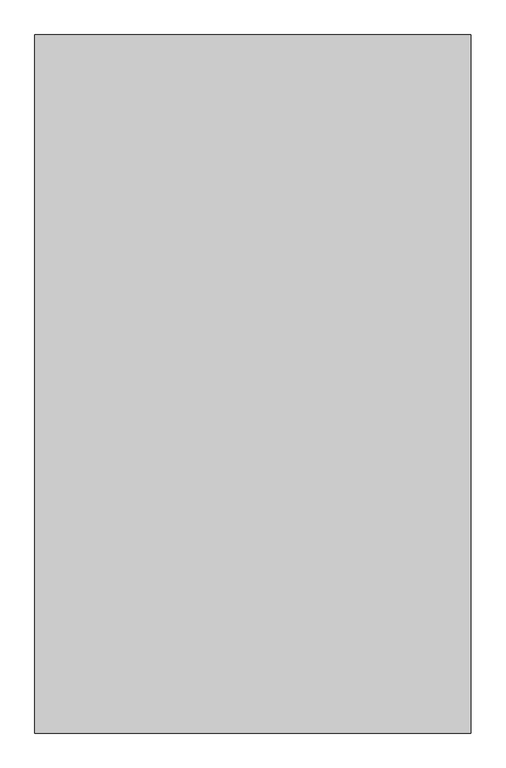
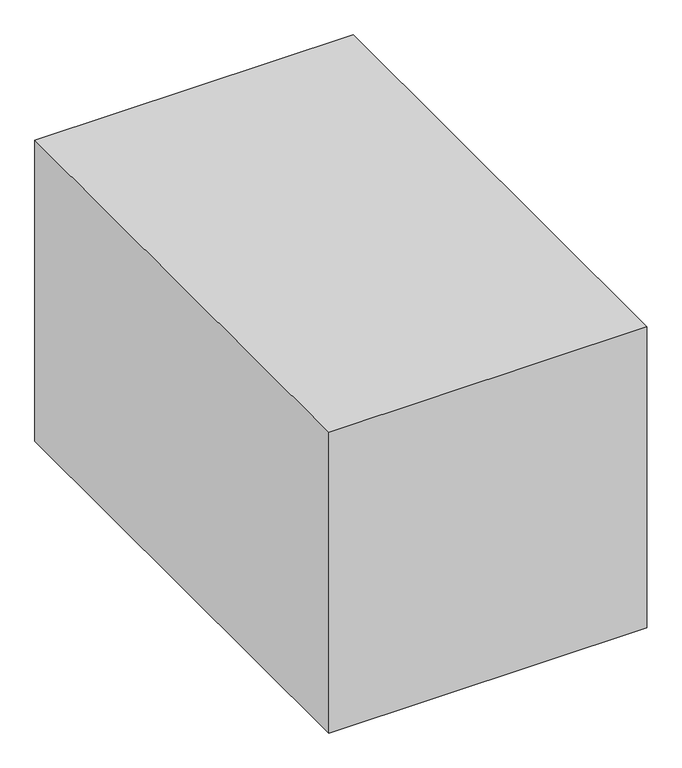
"""IFC4 building model written with IfcOpenShell, lengths in millimetres: proxy geometry, Space Planning Box_hec : Space Planning Box_hec."""

import ifcopenshell
import ifcopenshell.guid

model = None  # the IFC model being written
_history = None  # IfcOwnerHistory: only IFC2X3 demands one
_inside = {}  # id of a spatial element -> (the spatial element, [elements in it])
_under = {}  # id of a project, library or spatial element -> (it, [spatial elements below it])
_declared = {}  # id of a project -> (the project, [libraries it declares])
_typed = {}  # id of a type object -> (the type object, [elements of that type])
_made_of = {}  # id of a material, layer set ... -> (it, [elements and type objects made of it])


def new_model(schema):
    """Start an empty IFC model of exactly this schema.

    Asked for "IFC4X3", IfcOpenShell would pick the latest addendum, in which some entities
    have other attributes; the version numbers below select the first issue.
    IFC2X3 requires an IfcOwnerHistory on every rooted entity: one is made here for all.
    """
    global model, _history
    if schema == "IFC4X3":
        model = ifcopenshell.file(schema_version=(4, 3, 0, 0))
    else:
        model = ifcopenshell.file(schema=schema)
    _inside.clear()
    _under.clear()
    _declared.clear()
    _typed.clear()
    _made_of.clear()
    _history = None
    if model.schema == "IFC2X3":
        org = make("IfcOrganization", Name="unknown")
        user = make(
            "IfcPersonAndOrganization",
            ThePerson=make("IfcPerson", FamilyName="unknown"),
            TheOrganization=org,
        )
        app = make(
            "IfcApplication",
            ApplicationDeveloper=org,
            Version="unknown",
            ApplicationFullName="unknown",
            ApplicationIdentifier="unknown",
        )
        _history = make(
            "IfcOwnerHistory",
            OwningUser=user,
            OwningApplication=app,
            ChangeAction="ADDED",
            CreationDate=0,
        )
    return model


def make(cls, **values):
    """One entity of the class cls with the attributes given. An attribute that is None is left unset."""
    return model.create_entity(
        cls, **{name: value for name, value in values.items() if value is not None}
    )


def rooted(cls, **values):
    """An entity with a GlobalId (a new one), such as an element, a storey or a relation."""
    return make(cls, GlobalId=ifcopenshell.guid.new(), OwnerHistory=_history, **values)


def si_unit(unit_type, name, prefix=None):
    """IfcSIUnit, for example si_unit("LENGTHUNIT", "METRE", prefix="MILLI")."""
    return make("IfcSIUnit", UnitType=unit_type, Prefix=prefix, Name=name)


def assignment(units):
    """IfcUnitAssignment: the units of a project."""
    return None if units is None else make("IfcUnitAssignment", Units=units)


def point(xyz):
    """IfcCartesianPoint."""
    return None if xyz is None else make("IfcCartesianPoint", Coordinates=xyz)


def direction(xyz):
    """IfcDirection."""
    return None if xyz is None else make("IfcDirection", DirectionRatios=xyz)


def frame(location, z_axis=None, x_axis=None):
    """IfcAxis2Placement3D, a coordinate frame: its origin and axes. An axis left out is left unset."""
    return make(
        "IfcAxis2Placement3D",
        Location=point(location),
        Axis=direction(z_axis),
        RefDirection=direction(x_axis),
    )


def origin():
    """The frame at (0, 0, 0) with its axes left unset."""
    return frame((0.0, 0.0, 0.0))


def origin_with_axes():
    """The frame at (0, 0, 0) with the z axis (0, 0, 1) and the x axis (1, 0, 0) written out."""
    return frame((0.0, 0.0, 0.0), z_axis=(0.0, 0.0, 1.0), x_axis=(1.0, 0.0, 0.0))


def place(relative_to, where):
    """IfcLocalPlacement: puts the frame where relative to a parent placement (None: the world)."""
    return make(
        "IfcLocalPlacement", PlacementRelTo=relative_to, RelativePlacement=where
    )


def context(
    kind, dimensions, precision=None, world=None, true_north=None, identifier=None
):
    """IfcGeometricRepresentationContext, for example the 3D "Model" context."""
    return make(
        "IfcGeometricRepresentationContext",
        ContextIdentifier=identifier,
        ContextType=kind,
        CoordinateSpaceDimension=dimensions,
        Precision=precision,
        WorldCoordinateSystem=world,
        TrueNorth=true_north,
    )


def project(units=None, contexts=None):
    """IfcProject with its units and contexts."""
    return rooted(
        "IfcProject",
        Name="project",
        RepresentationContexts=contexts,
        UnitsInContext=assignment(units),
    )


def spatial(cls, under=None, at=None, **own):
    """A site, building, storey or space (cls), placed at a placement, below another one or the project."""
    s = rooted(cls, ObjectPlacement=at, **own)
    if under is not None:
        _under.setdefault(under.id(), (under, []))[1].append(s)
    return s


def polyline(points):
    """IfcPolyline through the points."""
    return make("IfcPolyline", Points=[point(p) for p in points])


def outline(outer, holes=None, kind="AREA"):
    """IfcArbitraryClosedProfileDef: a profile drawn as a closed curve; with holes, ...WithVoids."""
    if holes is None:
        return make("IfcArbitraryClosedProfileDef", ProfileType=kind, OuterCurve=outer)
    return make(
        "IfcArbitraryProfileDefWithVoids",
        ProfileType=kind,
        OuterCurve=outer,
        InnerCurves=holes,
    )


def extrude(swept, where, along, depth):
    """IfcExtrudedAreaSolid: the profile swept, set in the frame where, extruded along a direction by depth."""
    return make(
        "IfcExtrudedAreaSolid",
        SweptArea=swept,
        Position=where,
        ExtrudedDirection=direction(along),
        Depth=depth,
    )


def shape(context_of_items, identifier, shape_type, items):
    """IfcShapeRepresentation: the items that make up one representation, for example the "Body"."""
    return make(
        "IfcShapeRepresentation",
        ContextOfItems=context_of_items,
        RepresentationIdentifier=identifier,
        RepresentationType=shape_type,
        Items=items,
    )


def source(mapping_origin, context_of_items, identifier, shape_type, items):
    """IfcRepresentationMap: a shape defined once, which mapped items show again and again."""
    return make(
        "IfcRepresentationMap",
        MappingOrigin=mapping_origin,
        MappedRepresentation=shape(context_of_items, identifier, shape_type, items),
    )


def transform(
    local_origin,
    x_axis=None,
    y_axis=None,
    z_axis=None,
    scale=None,
    scale2=None,
    scale3=None,
    uniform=True,
):
    """IfcCartesianTransformationOperator3D, or its non-uniform kind. x_axis, y_axis, z_axis: its Axis1, 2, 3."""
    if uniform:
        return make(
            "IfcCartesianTransformationOperator3D",
            Axis1=direction(x_axis),
            Axis2=direction(y_axis),
            LocalOrigin=point(local_origin),
            Scale=scale,
            Axis3=direction(z_axis),
        )
    return make(
        "IfcCartesianTransformationOperator3DnonUniform",
        Axis1=direction(x_axis),
        Axis2=direction(y_axis),
        LocalOrigin=point(local_origin),
        Scale=scale,
        Axis3=direction(z_axis),
        Scale2=scale2,
        Scale3=scale3,
    )


def mapped(mapping_source, mapping_target):
    """IfcMappedItem: shows the shape of a source again, moved by a transform."""
    return make(
        "IfcMappedItem", MappingSource=mapping_source, MappingTarget=mapping_target
    )


def made_of(thing, what):
    """Note that an element or type object is made of a material, layer set ...; save() writes the relation."""
    if what is not None:
        _made_of.setdefault(what.id(), (what, []))[1].append(thing)
    return thing


def element(
    cls,
    number,
    at=None,
    inside=None,
    cuts=None,
    type_object=None,
    material=None,
    context=None,
    identifier="Body",
    shape_type=None,
    held_by="IfcProductDefinitionShape",
    body=None,
    shapes=None,
    **own,
):
    """One element of the class cls, such as IfcWall. Its Tag is "e" and its number.

    at: its placement. inside: the storey or other place that contains it. cuts: it is an
    opening in that element (IfcRelVoidsElement). A single representation is given by context,
    identifier, shape_type and body (its items); several are given by shapes. held_by: the class
    of the entity that holds the representations. save() writes the other relations.
    """
    e = rooted(cls, Tag="e%d" % number, ObjectPlacement=at, **own)
    if body is not None:
        shapes = [shape(context, identifier, shape_type, body)]
    if shapes is not None:
        e.Representation = make(held_by, Representations=shapes)
    if inside is not None:
        _inside.setdefault(inside.id(), (inside, []))[1].append(e)
    if cuts is not None:
        rooted(
            "IfcRelVoidsElement", RelatingBuildingElement=cuts, RelatedOpeningElement=e
        )
    if type_object is not None:
        _typed.setdefault(type_object.id(), (type_object, []))[1].append(e)
    return made_of(e, material)


def aggregate(whole, parts):
    """IfcRelAggregates: a whole, such as a stair, and the parts it consists of."""
    return rooted("IfcRelAggregates", RelatingObject=whole, RelatedObjects=parts)


def save(model, path):
    """Write the relations noted so far, then the file.

    IfcRelAggregates (storeys below a building ...), IfcRelContainedInSpatialStructure (elements
    in a storey), IfcRelDefinesByType, IfcRelAssociatesMaterial and IfcRelDeclares: one each for
    every whole, place, type object, material and project.
    """
    for whole, parts in _under.values():
        aggregate(whole, parts)
    for where, things in _inside.values():
        rooted(
            "IfcRelContainedInSpatialStructure",
            RelatedElements=things,
            RelatingStructure=where,
        )
    for kind, things in _typed.values():
        rooted("IfcRelDefinesByType", RelatedObjects=things, RelatingType=kind)
    for what, things in _made_of.values():
        rooted("IfcRelAssociatesMaterial", RelatedObjects=things, RelatingMaterial=what)
    for by, libraries in _declared.values():
        rooted("IfcRelDeclares", RelatingContext=by, RelatedDefinitions=libraries)
    model.write(path)


def generic_models_b37916ea(model_context):
    return source(origin(), model_context, "Body", "SweptSolid", [
        extrude(outline(polyline([(1750.0, 2800.0), (1750.0, -2800.0), (-1750.0, -2800.0), (-1750.0, 2800.0), (1750.0, 2800.0)])), origin_with_axes(), (0.0, 0.0, 1.0), 3500.0),
    ])


if __name__ == "__main__":
    model = new_model("IFC4")
    model_context = context("Model", 3, world=origin())
    ifc_project = project(units=[si_unit("LENGTHUNIT", "METRE", prefix="MILLI")], contexts=[model_context])
    site = spatial("IfcSite", under=ifc_project)
    building = spatial("IfcBuilding", under=site)
    placement = place(None, origin())
    generic_models_shape = generic_models_b37916ea(model_context)
    element("IfcBuildingElementProxy", 1, Name="Space Planning Box_hec : Space Planning Box_hec", ObjectType="Space Planning Box_hec : Space Planning Box_hec", at=placement, inside=building, context=model_context, shape_type="MappedRepresentation", body=[
        mapped(generic_models_shape, transform((0.0, 0.0, 0.0), x_axis=(1.0, 0.0, 0.0), y_axis=(0.0, 1.0, 0.0), z_axis=(0.0, 0.0, 1.0))),
    ])
    save(model, "model.ifc")

# Revit data of these elements
# Type "Space Planning Box_hec : Space Planning Box_hec"
#   Type Comments = "..."
#   Room Name [instance default] = "?"
#   Interior Finish [instance default] = ""
#   Exterior Finish [instance default] = ""
#   Department [instance default] = ""
#   Assembly Code = "..."
#   ceiling height [instance default] = 0
#   Width [instance default] = 1524 mm
#   Program Area [instance default] = 0.00 m²
#   Length [instance default] = 1524 mm
#   Height [instance default] = 1524 mm
#   Area [instance default] = 2.32258 m²
#   Fill Color [instance default] = Cyan
#   Default Elevation = 0
# Element 1 (IfcBuildingElementProxy, "Space Planning Box_hec : Space Planning Box_hec")
#   Room Name = "Toilet"
#   Exterior Finish = "RF1..N/A,,N/A..N/A..N/A"
#   Department = "AR"
#   Width = 3500 mm
#   Program Area = 19.60 m²
#   Length = 5600 mm
#   Height = 3500 mm
#   Area = 19.60 m²
#   Materials on its faces: "Cyan"
# Materials
#   "Cyan": class "Generic", colour RGB 0 255 255, transparency 0.2, Cost = 0
